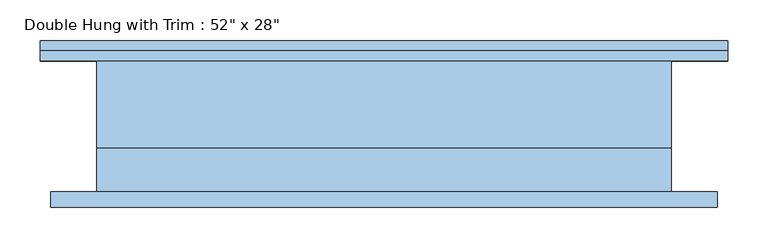
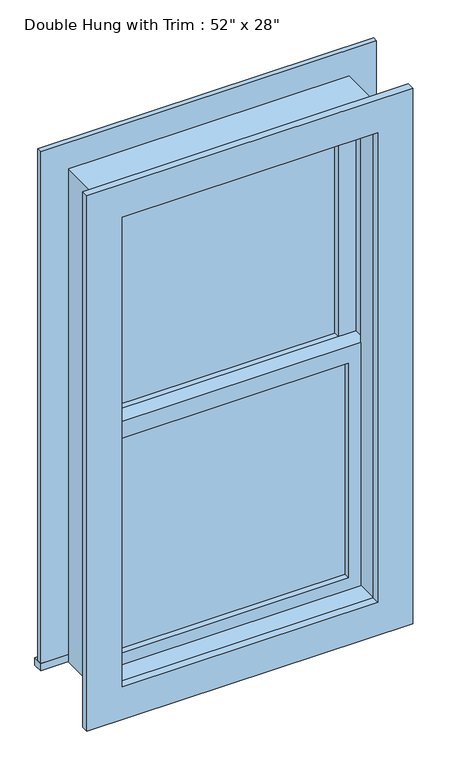
"""IFC4 building model written with IfcOpenShell, lengths in millimetres: window geometry."""

from ifc_helpers import new_model, si_unit, frame, origin, place, context, project, spatial, polyline, outline, extrude, source, transform, mapped, element, save


def window_ca4ad738(model_context):
    return source(origin(), model_context, "Body", "SweptSolid", [
        extrude(outline(polyline([(-292.1, 1.5875), (292.1, 1.5875), (292.1, -11.1125), (-292.1, -11.1125), (-292.1, 1.5875)])), frame((0.0, 0.0, 571.5), z_axis=(0.0, 0.0, 1.0), x_axis=(1.0, 0.0, 0.0)), (0.0, 0.0, 1.0), 574.675),
        extrude(outline(polyline([(1190.625, -336.55), (527.05, -336.55), (527.05, 336.55), (1190.625, 336.55), (1190.625, -336.55)]), holes=[polyline([(1146.175, -292.1), (1146.175, 292.1), (571.5, 292.1), (571.5, -292.1), (1146.175, -292.1)])]), frame((0.0, -26.9875, 0.0), z_axis=(0.0, 1.0, 0.0), x_axis=(0.0, 0.0, 1.0)), (0.0, 0.0, 1.0), 44.45),
        extrude(outline(polyline([(-425.45, 106.3625), (425.45, 106.3625), (425.45, 80.9625), (-425.45, 80.9625), (-425.45, 106.3625)])), frame((0.0, 0.0, 508.0), z_axis=(0.0, 0.0, 1.0), x_axis=(1.0, 0.0, 0.0)), (0.0, 0.0, 1.0), 19.05),
        extrude(outline(polyline([(1809.75, -336.55), (1809.75, 336.55), (527.05, 336.55), (527.05, 425.45), (1898.65, 425.45), (1898.65, -425.45), (527.05, -425.45), (527.05, -336.55), (1809.75, -336.55)])), frame((0.0, 80.9625, 0.0), z_axis=(0.0, 1.0, 0.0), x_axis=(0.0, 0.0, 1.0)), (0.0, 0.0, 1.0), 12.7),
        extrude(outline(polyline([(1885.95, 412.75), (1885.95, -412.75), (450.85, -412.75), (450.85, 412.75), (1885.95, 412.75)]), holes=[polyline([(1797.05, 323.85), (539.75, 323.85), (539.75, -323.85), (1797.05, -323.85), (1797.05, 323.85)])]), frame((0.0, -100.0125, 0.0), z_axis=(0.0, 1.0, 0.0), x_axis=(0.0, 0.0, 1.0)), (0.0, 0.0, 1.0), 19.05),
        extrude(outline(polyline([(292.1, 33.3375), (-292.1, 33.3375), (-292.1, 46.0375), (292.1, 46.0375), (292.1, 33.3375)])), frame((0.0, 0.0, 1190.625), z_axis=(0.0, 0.0, 1.0), x_axis=(1.0, 0.0, 0.0)), (0.0, 0.0, 1.0), 574.675),
        extrude(outline(polyline([(1809.75, -336.55), (1146.175, -336.55), (1146.175, 336.55), (1809.75, 336.55), (1809.75, -336.55)]), holes=[polyline([(1765.3, -292.1), (1765.3, 292.1), (1190.625, 292.1), (1190.625, -292.1), (1765.3, -292.1)])]), frame((0.0, 17.4625, 0.0), z_axis=(0.0, 1.0, 0.0), x_axis=(0.0, 0.0, 1.0)), (0.0, 0.0, 1.0), 44.45),
        extrude(outline(polyline([(1828.8, -355.6), (508.0, -355.6), (508.0, 355.6), (1828.8, 355.6), (1828.8, -355.6)]), holes=[polyline([(1797.05, -323.85), (1797.05, 323.85), (539.75, 323.85), (539.75, -323.85), (1797.05, -323.85)])]), frame((0.0, -80.9625, 0.0), z_axis=(0.0, 1.0, 0.0), x_axis=(0.0, 0.0, 1.0)), (0.0, 0.0, 1.0), 53.975),
        extrude(outline(polyline([(1828.8, 355.6), (1828.8, -355.6), (508.0, -355.6), (508.0, 355.6), (1828.8, 355.6)]), holes=[polyline([(1809.75, 336.55), (527.05, 336.55), (527.05, -336.55), (1809.75, -336.55), (1809.75, 336.55)])]), frame((0.0, -26.9875, 0.0), z_axis=(0.0, 1.0, 0.0), x_axis=(0.0, 0.0, 1.0)), (0.0, 0.0, 1.0), 107.95),
    ])


if __name__ == "__main__":
    model = new_model("IFC4")
    model_context = context("Model", 3, world=origin())
    ifc_project = project(units=[si_unit("LENGTHUNIT", "METRE", prefix="MILLI")], contexts=[model_context])
    site = spatial("IfcSite", under=ifc_project)
    building = spatial("IfcBuilding", under=site)
    placement = place(None, origin())
    window_shape = window_ca4ad738(model_context)
    element("IfcWindow", 1, ObjectType="Double Hung with Trim : 52\" x 28\"", at=placement, inside=building, context=model_context, shape_type="MappedRepresentation", body=[
        mapped(window_shape, transform((0.0, 0.0, 0.0), x_axis=(1.0, 0.0, 0.0), y_axis=(0.0, 1.0, 0.0), z_axis=(0.0, 0.0, 1.0))),
    ])
    save(model, "model.ifc")

# Revit data of these elements
# Type "Double Hung with Trim : 52\" x 28\""
#   Type Mark = "42"
#   COBie.Type.CreatedBy = "doug.wood@us.ibm.com"
#   COBie.Type.CreatedOn = "2016-04-14T02:07:26"
#   COBie.Type.Name = "Windows_Double Hung with Trim_52\" x 28\"_42"
#   COBie.Type.Category = "23-30 20 17 17 14 : Double-Hung Windows"
#   COBie.Type.Description = "Double Hung with Trim_52\" x 28\""
#   COBie.Type.Manufacturer = ""
#   COBie.Type.ModelNumber = ""
#   Construction Type Id = "GSP4R"
#   Assembly Code = "B2020100"
#   Analytic Construction = "1/8 in Pilkington single glazing"
#   COBie.Type.ReplacementCost = 0
#   Visual Light Transmittance = 0.9
#   Solar Heat Gain Coefficient = 0.78
#   Heat Transfer Coefficient (U) = 3.6886 W/(m²·K)
#   Height = 4' - 4"
#   Default Sill Height = 1' - 8"
#   Trim Projection - Ext. = 0' - 0 1/2"
#   Trim Projection - Int. = 0' - 0 3/4"
#   Trim Width - Exterior = 0' - 3 1/2"
#   Trim Width - Interior = 0' - 3 1/2"
#   Width = 2' - 4"
#   Window Inset = 0' - 0 3/4"
#   COBie.Type = no
#   Glass Pane Material = Glass
#   Sash Material = Sash - White
#   Trim Exterior Material = Trim - White
#   Trim Interior Material = Trim - White
#   Wall Closure = (empty or 0)
# Element 1 (IfcWindow, "Double Hung with Trim : 52\" x 28\"")
#   Materials on its faces: "Sash - White", "Trim - White", "Glass"
# Materials
#   "Glass": class "Glass", colour RGB 0 128 192, transparency 0.75, Description = "Soda Lime Glass", Cost = 0
#   "Sash - White": class "Wood", colour RGB 255 255 255, transparency 0, Cost = 0
#   "Trim - White": class "Wood", colour RGB 255 255 255, transparency 0, Cost = 0
